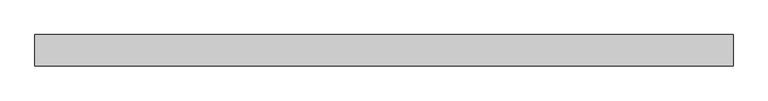
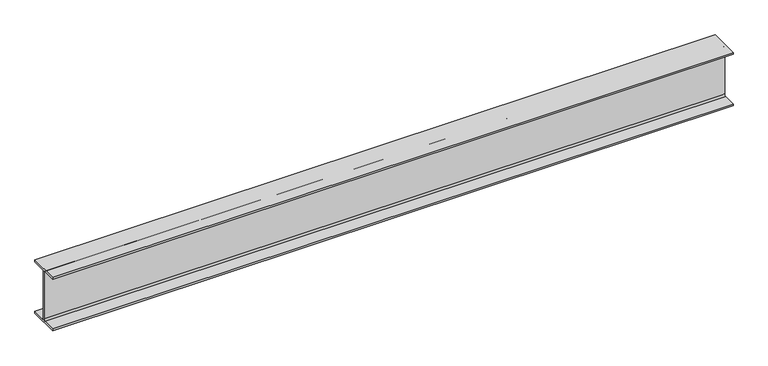
"""IFC4 building model written with IfcOpenShell, lengths in millimetres: beam geometry, Steel Beam_H-KSD3502 : H_SB_ASB_H-200x200x8x12."""

from ifc_helpers import new_model, si_unit, point, frame, frame_2d, origin, place, context, project, spatial, polyline, circle_curve, trimmed, segment, composite_curve, outline, extrude, source, transform, mapped, element, save


def beam_298d0fa7(model_context):
    return source(origin(), model_context, "Body", "SweptSolid", [
        extrude(outline(composite_curve([segment(polyline([(-82.5, -141.5), (-11.9, -141.5)]), True, "CONTINUOUS"), segment(trimmed(circle_curve(frame_2d((-11.9, -132.6)), 8.9), [point((-11.9, -141.5))], [point((-3.0, -132.6))], True, "CARTESIAN"), True, "CONTINUOUS"), segment(polyline([(-3.0, -132.6), (-3.0, 132.6)]), True, "CONTINUOUS"), segment(trimmed(circle_curve(frame_2d((-11.9, 132.6)), 8.9), [point((-3.0, 132.6))], [point((-11.9, 141.5))], True, "CARTESIAN"), True, "CONTINUOUS"), segment(polyline([(-11.9, 141.5), (-82.5, 141.5), (-82.5, 151.7), (82.5, 151.7), (82.5, 141.5), (11.9, 141.5)]), True, "CONTINUOUS"), segment(trimmed(circle_curve(frame_2d((11.9, 132.6)), 8.9), [point((11.9, 141.5))], [point((3.0, 132.6))], True, "CARTESIAN"), True, "CONTINUOUS"), segment(polyline([(3.0, 132.6), (3.0, -132.6)]), True, "CONTINUOUS"), segment(trimmed(circle_curve(frame_2d((11.9, -132.6)), 8.9), [point((3.0, -132.6))], [point((11.9, -141.5))], True, "CARTESIAN"), True, "CONTINUOUS"), segment(polyline([(11.9, -141.5), (82.5, -141.5), (82.5, -151.7), (-82.5, -151.7), (-82.5, -141.5)]), True, "CONTINUOUS")], self_intersect=False)), frame((-1840.6096779, 0.0, 0.0), z_axis=(1.0, 0.0, 0.0), x_axis=(0.0, 1.0, 0.0)), (0.0, 0.0, 1.0), 3657.360877),
    ])


if __name__ == "__main__":
    model = new_model("IFC4")
    model_context = context("Model", 3, world=origin())
    ifc_project = project(units=[si_unit("LENGTHUNIT", "METRE", prefix="MILLI")], contexts=[model_context])
    site = spatial("IfcSite", under=ifc_project)
    building = spatial("IfcBuilding", under=site)
    placement = place(None, origin())
    beam_shape = beam_298d0fa7(model_context)
    element("IfcBeam", 1, ObjectType="Steel Beam_H-KSD3502 : H_SB_ASB_H-200x200x8x12", at=placement, inside=building, context=model_context, shape_type="MappedRepresentation", body=[
        mapped(beam_shape, transform((0.0, 0.0, 0.0), x_axis=(1.0, 0.0, 0.0), y_axis=(0.0, 1.0, 0.0), z_axis=(0.0, 0.0, 1.0))),
    ])
    save(model, "model.ifc")

# Revit data of these elements
# Type "Steel Beam_H-KSD3502 : H_SB_ASB_H-200x200x8x12"
#   Width = 20.0 cm
#   Web Thickness = 0.8 cm
#   Web Fillet = 1.3 cm
#   Warping Constant = 141376.0 cm⁶
#   Torsional Moment of Inertia = 26.2485 cm⁴
#   Torsional Modulus = 1.0 cm³
#   Section Area = 63.53 cm²
#   Plastic Modulus weak axis = 244.0 cm³
#   Plastic Modulus strong axis = 525.0 cm³
#   Perimeter = 1.16 m²/m
#   Nominal Weight = 49.90 kgf/m
#   Moment of Inertia weak axis = 1600.00 cm⁴
#   Moment of Inertia strong axis = 4720.00 cm⁴
#   Height = 20.0 cm
#   Flange Thickness = 1.2 cm
#   Elastic Modulus weak axis = 160.0 cm³
#   Elastic Modulus strong axis = 472.0 cm³
#   Centroid Vertical = 10.0 cm
#   Centroid Horizontal = 10.0 cm
#   Length [instance default] = 1.5240 m
#   Structural Material [instance default] = Steel, 45-345
#   Assembly Code = ""
# Element 1 (IfcBeam, "Steel Beam_H-KSD3502 : H_SB_ASB_H-200x200x8x12")
#   Structural Material = none
# Materials
#   "Steel, 45-345": class "Metal", colour RGB 189 187 185, transparency 0, Description = "Steel 345 MPa", Cost = 0
